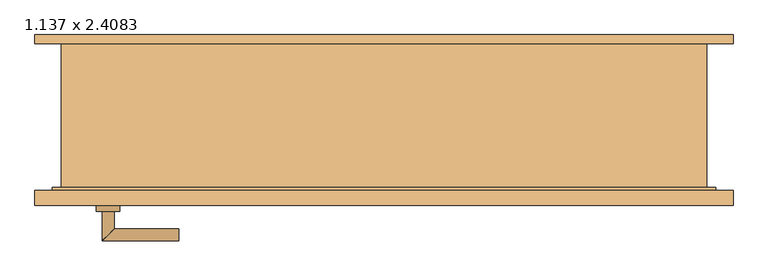
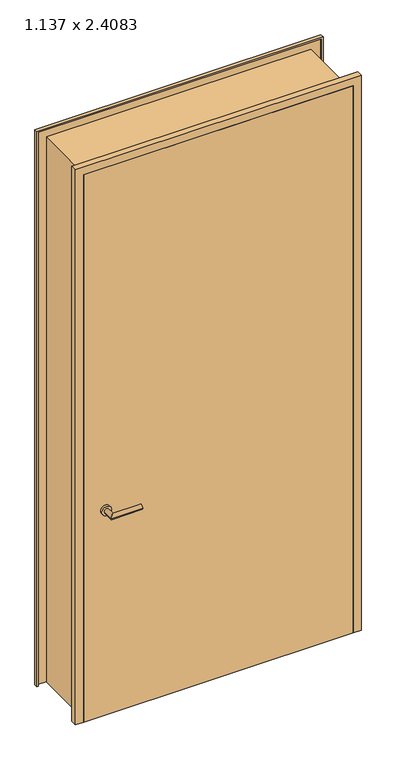
"""IFC4 building model written with IfcOpenShell, lengths in millimetres: door geometry, Drehflügel 1-flg - Stahlzarge : 1.137 x 2.4083."""

from ifc_helpers import new_model, si_unit, point, frame, frame_2d, origin, place, context, project, spatial, polyline, circle_curve, ellipse_curve, trimmed, segment, composite_curve, outline, extrude, faceted_brep, source, transform, mapped, element, save
from ifc_brep_helpers import plane_surface, cylinder_surface, advanced_brep


def door_1_137_x_2_4083_578afda8(model_context):
    return source(origin(), model_context, "Body", "SolidModel", [
        advanced_brep(
        [(-478.5, -114.4346141, 915.0), (-458.5, -114.4346141, 915.0), (-458.5, -64.4346141, 915.0), (-478.5, -44.4346141, 915.0), (-348.5, -44.4346141, 915.0), (-348.5, -64.4346141, 915.0)],
        [
            (0, 1, circle_curve(frame((-468.5, -114.4346141, 915.0), z_axis=(0.0, -1.0, 0.0), x_axis=(1.0, 0.0, 0.0)), 10.0)),
            (1, 0, circle_curve(frame((-468.5, -114.4346141, 915.0), z_axis=(0.0, -1.0, 0.0), x_axis=(1.0, 0.0, 0.0)), 10.0)),
            (1, 2),
            (2, 3, ellipse_curve(frame((-468.5, -54.4346141, 915.0), z_axis=(-0.7071067811865385, -0.7071067811865565, 0.0), x_axis=(0.7071067811865563, -0.7071067811865386, 0.0)), 14.1421356, 10.0)),
            (3, 0),
            (3, 2, ellipse_curve(frame((-468.5, -54.4346141, 915.0), z_axis=(-0.7071067811865385, -0.7071067811865565, 0.0), x_axis=(0.7071067811865563, -0.7071067811865386, 0.0)), 14.1421356, 10.0)),
            (4, 5, circle_curve(frame((-348.5, -54.4346141, 915.0), z_axis=(1.0, 0.0, 0.0), x_axis=(0.0, -1.0, 0.0)), 10.0)),
            (5, 4, circle_curve(frame((-348.5, -54.4346141, 915.0), z_axis=(1.0, 0.0, 0.0), x_axis=(0.0, -1.0, 0.0)), 10.0)),
            (2, 5),
            (4, 3),
        ],
        [
            plane_surface(frame((-468.5, -114.4346141, -372.7526403), z_axis=(0.0, -1.0, 0.0), x_axis=(0.0, 0.0, 1.0))),
            cylinder_surface(frame((-468.5, -114.4346141, 915.0), z_axis=(0.0, -1.0, 0.0), x_axis=(1.0, 0.0, 0.0)), 10.0),
            plane_surface(frame((-348.5, -54.4346141, -372.7526403), z_axis=(1.0, 0.0, 0.0), x_axis=(0.0, 0.0, 1.0))),
            cylinder_surface(frame((-468.5, -54.4346141, 915.0), z_axis=(-1.0, 0.0, 0.0), x_axis=(0.0, -1.0, 0.0)), 10.0),
        ],
        [
            (0, [[1, 2]]),
            (1, [[3, 4, 5, -2]]),
            (1, [[-5, 6, -3, -1]]),
            (2, [[7, 8]]),
            (3, [[9, -7, 10, -4]]),
            (3, [[-10, -8, -9, -6]]),
        ],
    ),
        advanced_brep(
        [(-458.5, -174.4346141, 915.0), (-478.5, -174.4346141, 915.0), (-478.5, -224.4346141, 915.0), (-458.5, -204.4346141, 915.0), (-348.5, -204.4346141, 915.0), (-348.5, -224.4346141, 915.0)],
        [
            (0, 1, circle_curve(frame((-468.5, -174.4346141, 915.0), z_axis=(0.0, 1.0, 0.0), x_axis=(-1.0, 0.0, 0.0)), 10.0)),
            (1, 0, circle_curve(frame((-468.5, -174.4346141, 915.0), z_axis=(0.0, 1.0, 0.0), x_axis=(-1.0, 0.0, 0.0)), 10.0)),
            (1, 2),
            (2, 3, ellipse_curve(frame((-468.5, -214.4346141, 915.0), z_axis=(-0.7071067811865475, 0.7071067811865475, 0.0), x_axis=(0.7071067811865474, 0.7071067811865476, 0.0)), 14.1421356, 10.0)),
            (3, 0),
            (3, 2, ellipse_curve(frame((-468.5, -214.4346141, 915.0), z_axis=(-0.7071067811865475, 0.7071067811865475, 0.0), x_axis=(0.7071067811865474, 0.7071067811865476, 0.0)), 14.1421356, 10.0)),
            (4, 5, circle_curve(frame((-348.5, -214.4346141, 915.0), z_axis=(1.0, 0.0, 0.0), x_axis=(0.0, -1.0, 0.0)), 10.0)),
            (5, 4, circle_curve(frame((-348.5, -214.4346141, 915.0), z_axis=(1.0, 0.0, 0.0), x_axis=(0.0, -1.0, 0.0)), 10.0)),
            (2, 5),
            (4, 3),
        ],
        [
            plane_surface(frame((-468.5, -174.4346141, -372.7526403), z_axis=(0.0, 1.0, 0.0), x_axis=(0.0, 0.0, 1.0))),
            cylinder_surface(frame((-468.5, -174.4346141, 915.0), z_axis=(0.0, 1.0, 0.0), x_axis=(-1.0, 0.0, 0.0)), 10.0),
            plane_surface(frame((-348.5, -214.4346141, -372.7526403), z_axis=(1.0, 0.0, 0.0), x_axis=(0.0, 0.0, 1.0))),
            cylinder_surface(frame((-468.5, -214.4346141, 915.0), z_axis=(-1.0, 0.0, 0.0), x_axis=(0.0, -1.0, 0.0)), 10.0),
        ],
        [
            (0, [[1, 2]]),
            (1, [[3, 4, 5, -2]]),
            (1, [[-5, 6, -3, -1]]),
            (2, [[7, 8]]),
            (3, [[9, -7, 10, -4]]),
            (3, [[-10, -8, -9, -6]]),
        ],
    ),
        extrude(outline(composite_curve([segment(trimmed(circle_curve(frame_2d((915.0, -468.5)), 20.0), [point((915.0, -488.5))], [point((915.0, -448.5))], False, "CARTESIAN"), True, "CONTINUOUS"), segment(trimmed(circle_curve(frame_2d((915.0, -468.5)), 20.0), [point((915.0, -448.5))], [point((915.0, -488.5))], False, "CARTESIAN"), True, "CONTINUOUS")], self_intersect=False)), frame((0.0, -114.4346141, 0.0), z_axis=(0.0, 1.0, 0.0), x_axis=(0.0, 0.0, 1.0)), (0.0, 0.0, 1.0), 10.0),
        extrude(outline(composite_curve([segment(trimmed(circle_curve(frame_2d((915.0, -468.5)), 20.0), [point((915.0, -488.5))], [point((915.0, -448.5))], False, "CARTESIAN"), True, "CONTINUOUS"), segment(trimmed(circle_curve(frame_2d((915.0, -468.5)), 20.0), [point((915.0, -448.5))], [point((915.0, -488.5))], False, "CARTESIAN"), True, "CONTINUOUS")], self_intersect=False)), frame((0.0, -174.4346141, 0.0), z_axis=(0.0, 1.0, 0.0), x_axis=(0.0, 0.0, 1.0)), (0.0, 0.0, 1.0), 10.0),
        extrude(outline(polyline([(558.5, -139.4346141), (558.5, -164.4346141), (-558.5, -164.4346141), (-558.5, -139.4346141), (558.5, -139.4346141)])), frame((0.0, 0.0, 15.0), z_axis=(0.0, 0.0, 1.0), x_axis=(1.0, 0.0, 0.0)), (0.0, 0.0, 1.0), 2398.3),
        faceted_brep([(592.9603207, 125.5653859, 15.0), (592.9603207, 110.5653859, 15.0), (587.9603207, 110.5653859, 15.0), (587.9603207, 120.5653859, 15.0), (548.5, 120.5653859, 15.0), (548.5, -134.4346141, 15.0), (563.5, -134.4346141, 15.0), (563.5, -159.4346141, 15.0), (587.9603207, -159.4346141, 15.0), (587.9603207, -139.4346141, 15.0), (592.9603207, -139.4346141, 15.0), (592.9603207, -164.4346141, 15.0), (558.5, -164.4346141, 15.0), (558.5, -139.4346141, 15.0), (543.5, -139.4346141, 15.0), (543.5, 125.5653859, 15.0), (543.5, 125.5653859, 2398.3), (-543.5, 125.5653859, 2398.3), (-543.5, 125.5653859, 15.0), (-592.9603207, 125.5653859, 15.0), (-592.9603207, 125.5653859, 2447.7603207), (592.9603207, 125.5653859, 2447.7603207), (543.5, -139.4346141, 2398.3), (558.5, -139.4346141, 2413.3), (-558.5, -139.4346141, 2413.3), (-558.5, -139.4346141, 15.0), (-543.5, -139.4346141, 15.0), (-543.5, -139.4346141, 2398.3), (558.5, -164.4346141, 2413.3), (592.9603207, -164.4346141, 2447.7603207), (-592.9603207, -164.4346141, 2447.7603207), (-592.9603207, -164.4346141, 15.0), (-558.5, -164.4346141, 15.0), (-558.5, -164.4346141, 2413.3), (592.9603207, -139.4346141, 2447.7603207), (587.9603207, -139.4346141, 2442.7603207), (-587.9603207, -139.4346141, 2442.7603207), (-587.9603207, -139.4346141, 15.0), (-592.9603207, -139.4346141, 15.0), (-592.9603207, -139.4346141, 2447.7603207), (587.9603207, -159.4346141, 2442.7603207), (563.5, -159.4346141, 2418.3), (-563.5, -159.4346141, 2418.3), (-563.5, -159.4346141, 15.0), (-587.9603207, -159.4346141, 15.0), (-587.9603207, -159.4346141, 2442.7603207), (563.5, -134.4346141, 2418.3), (548.5, -134.4346141, 2403.3), (-548.5, -134.4346141, 2403.3), (-548.5, -134.4346141, 15.0), (-563.5, -134.4346141, 15.0), (-563.5, -134.4346141, 2418.3), (548.5, 120.5653859, 2403.3), (587.9603207, 120.5653859, 2442.7603207), (-587.9603207, 120.5653859, 2442.7603207), (-587.9603207, 120.5653859, 15.0), (-548.5, 120.5653859, 15.0), (-548.5, 120.5653859, 2403.3), (587.9603207, 110.5653859, 2442.7603207), (592.9603207, 110.5653859, 2447.7603207), (-592.9603207, 110.5653859, 2447.7603207), (-592.9603207, 110.5653859, 15.0), (-587.9603207, 110.5653859, 15.0), (-587.9603207, 110.5653859, 2442.7603207)], [[[0, 1, 2, 3, 4, 5, 6, 7, 8, 9, 10, 11, 12, 13, 14, 15]], [[15, 16, 17, 18, 19, 20, 21, 0]], [[14, 22, 16, 15]], [[13, 23, 24, 25, 26, 27, 22, 14]], [[12, 28, 23, 13]], [[11, 29, 30, 31, 32, 33, 28, 12]], [[10, 34, 29, 11]], [[9, 35, 36, 37, 38, 39, 34, 10]], [[8, 40, 35, 9]], [[7, 41, 42, 43, 44, 45, 40, 8]], [[6, 46, 41, 7]], [[5, 47, 48, 49, 50, 51, 46, 6]], [[4, 52, 47, 5]], [[3, 53, 54, 55, 56, 57, 52, 4]], [[2, 58, 53, 3]], [[1, 59, 60, 61, 62, 63, 58, 2]], [[0, 21, 59, 1]], [[20, 19, 61, 60]], [[19, 18, 26, 25, 32, 31, 38, 37, 44, 43, 50, 49, 56, 55, 62, 61]], [[27, 26, 18, 17]], [[33, 32, 25, 24]], [[39, 38, 31, 30]], [[45, 44, 37, 36]], [[51, 50, 43, 42]], [[57, 56, 49, 48]], [[63, 62, 55, 54]], [[22, 27, 17, 16]], [[28, 33, 24, 23]], [[34, 39, 30, 29]], [[40, 45, 36, 35]], [[46, 51, 42, 41]], [[52, 57, 48, 47]], [[58, 63, 54, 53]], [[21, 20, 60, 59]]]),
    ])


if __name__ == "__main__":
    model = new_model("IFC4")
    model_context = context("Model", 3, world=origin())
    ifc_project = project(units=[si_unit("LENGTHUNIT", "METRE", prefix="MILLI")], contexts=[model_context])
    site = spatial("IfcSite", under=ifc_project)
    building = spatial("IfcBuilding", under=site)
    placement = place(None, origin())
    door_1_137_x_2_4083_shape = door_1_137_x_2_4083_578afda8(model_context)
    element("IfcDoor", 1, ObjectType="Drehflügel 1-flg - Stahlzarge : 1.137 x 2.4083", at=placement, inside=building, context=model_context, shape_type="MappedRepresentation", body=[
        mapped(door_1_137_x_2_4083_shape, transform((0.0, 0.0, 0.0), x_axis=(1.0, 0.0, 0.0), y_axis=(0.0, 1.0, 0.0), z_axis=(0.0, 0.0, 1.0))),
    ])
    save(model, "model.ifc")

# Revit data of these elements
# Type "Drehflügel 1-flg - Stahlzarge : 1.137 x 2.4083"
#   Type Mark = "21"
#   Operation = "SingleSwingRight"
#   Keynote = "16.03"
#   Analytic Construction = "Metall"
#   Thermal Resistance (R) = 0.270117 (m²·K)/W
#   Heat Transfer Coefficient (U) = 3.7021 W/(m²·K)
#   Rough Width = 1.137 m
#   Rough Height [instance default] = 2.5083 m
#   Höhe Türgriff [instance default] = 0.900 m
#   Height = 2.4083 m
#   Fußbodenaufbau [instance default] = 0.100 m
#   Width = 1.137 m
#   Sichtbarkeit Sturzlinien [instance default] = yes
#   Türgriff auswählen [instance default] = element 221079
#   Türgriff [instance default] = none
#   Türflügel [instance default] = none
#   Rahmen/Pfosten [instance default] = Metall - Lackiert - Grau
#   Visual Light Transmittance = 0
#   Solar Heat Gain Coefficient = 0
#   Function = (empty or 0)
#   Wall Closure = (empty or 0)
# Element 1 (IfcDoor, "Drehflügel 1-flg - Stahlzarge : 1.137 x 2.4083")
#   Rough Height = 2.4233 m
#   Fußbodenaufbau = 0.015 m
#   Materials on its faces: "Metall - Lackiert - Grau", "Metall - Chrom", "Holz - Birke"
# Materials
#   "Metall - Lackiert - Grau": class "Farbe 1", colour RGB 98 98 98, transparency 0, Cost = 0
#   "Metall - Chrom": class "Metall", colour RGB 247 247 247, transparency 0, Cost = 0
#   "Holz - Birke": class "Holz", colour RGB 213 164 103, transparency 0, Cost = 0
